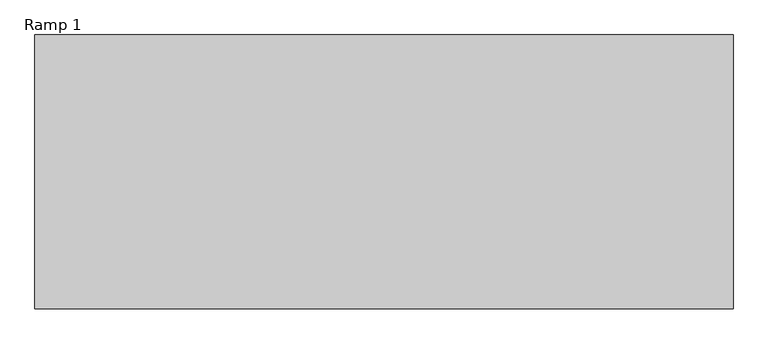
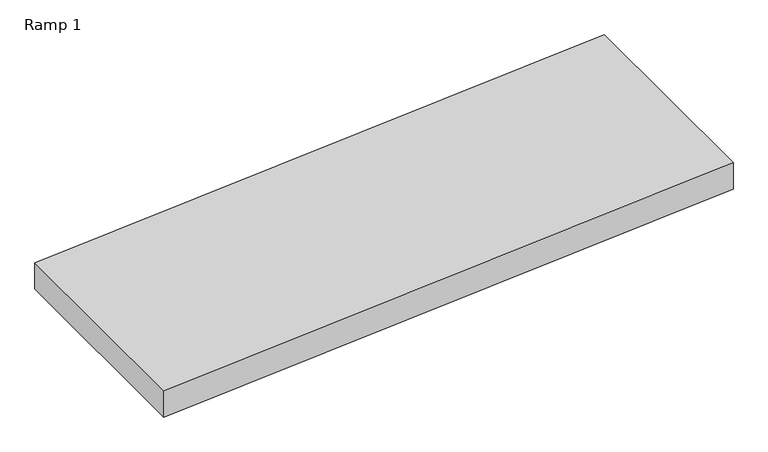
"""IFC4 building model written with IfcOpenShell, lengths in millimetres: ramp geometry, Ramp 1."""

import ifcopenshell
import ifcopenshell.guid

model = None  # the IFC model being written
_history = None  # IfcOwnerHistory: only IFC2X3 demands one
_inside = {}  # id of a spatial element -> (the spatial element, [elements in it])
_under = {}  # id of a project, library or spatial element -> (it, [spatial elements below it])
_declared = {}  # id of a project -> (the project, [libraries it declares])
_typed = {}  # id of a type object -> (the type object, [elements of that type])
_made_of = {}  # id of a material, layer set ... -> (it, [elements and type objects made of it])


def new_model(schema):
    """Start an empty IFC model of exactly this schema.

    Asked for "IFC4X3", IfcOpenShell would pick the latest addendum, in which some entities
    have other attributes; the version numbers below select the first issue.
    IFC2X3 requires an IfcOwnerHistory on every rooted entity: one is made here for all.
    """
    global model, _history
    if schema == "IFC4X3":
        model = ifcopenshell.file(schema_version=(4, 3, 0, 0))
    else:
        model = ifcopenshell.file(schema=schema)
    _inside.clear()
    _under.clear()
    _declared.clear()
    _typed.clear()
    _made_of.clear()
    _history = None
    if model.schema == "IFC2X3":
        org = make("IfcOrganization", Name="unknown")
        user = make(
            "IfcPersonAndOrganization",
            ThePerson=make("IfcPerson", FamilyName="unknown"),
            TheOrganization=org,
        )
        app = make(
            "IfcApplication",
            ApplicationDeveloper=org,
            Version="unknown",
            ApplicationFullName="unknown",
            ApplicationIdentifier="unknown",
        )
        _history = make(
            "IfcOwnerHistory",
            OwningUser=user,
            OwningApplication=app,
            ChangeAction="ADDED",
            CreationDate=0,
        )
    return model


def make(cls, **values):
    """One entity of the class cls with the attributes given. An attribute that is None is left unset."""
    return model.create_entity(
        cls, **{name: value for name, value in values.items() if value is not None}
    )


def rooted(cls, **values):
    """An entity with a GlobalId (a new one), such as an element, a storey or a relation."""
    return make(cls, GlobalId=ifcopenshell.guid.new(), OwnerHistory=_history, **values)


def si_unit(unit_type, name, prefix=None):
    """IfcSIUnit, for example si_unit("LENGTHUNIT", "METRE", prefix="MILLI")."""
    return make("IfcSIUnit", UnitType=unit_type, Prefix=prefix, Name=name)


def assignment(units):
    """IfcUnitAssignment: the units of a project."""
    return None if units is None else make("IfcUnitAssignment", Units=units)


def point(xyz):
    """IfcCartesianPoint."""
    return None if xyz is None else make("IfcCartesianPoint", Coordinates=xyz)


def direction(xyz):
    """IfcDirection."""
    return None if xyz is None else make("IfcDirection", DirectionRatios=xyz)


def frame(location, z_axis=None, x_axis=None):
    """IfcAxis2Placement3D, a coordinate frame: its origin and axes. An axis left out is left unset."""
    return make(
        "IfcAxis2Placement3D",
        Location=point(location),
        Axis=direction(z_axis),
        RefDirection=direction(x_axis),
    )


def origin():
    """The frame at (0, 0, 0) with its axes left unset."""
    return frame((0.0, 0.0, 0.0))


def place(relative_to, where):
    """IfcLocalPlacement: puts the frame where relative to a parent placement (None: the world)."""
    return make(
        "IfcLocalPlacement", PlacementRelTo=relative_to, RelativePlacement=where
    )


def context(
    kind, dimensions, precision=None, world=None, true_north=None, identifier=None
):
    """IfcGeometricRepresentationContext, for example the 3D "Model" context."""
    return make(
        "IfcGeometricRepresentationContext",
        ContextIdentifier=identifier,
        ContextType=kind,
        CoordinateSpaceDimension=dimensions,
        Precision=precision,
        WorldCoordinateSystem=world,
        TrueNorth=true_north,
    )


def project(units=None, contexts=None):
    """IfcProject with its units and contexts."""
    return rooted(
        "IfcProject",
        Name="project",
        RepresentationContexts=contexts,
        UnitsInContext=assignment(units),
    )


def spatial(cls, under=None, at=None, **own):
    """A site, building, storey or space (cls), placed at a placement, below another one or the project."""
    s = rooted(cls, ObjectPlacement=at, **own)
    if under is not None:
        _under.setdefault(under.id(), (under, []))[1].append(s)
    return s


def polyline(points):
    """IfcPolyline through the points."""
    return make("IfcPolyline", Points=[point(p) for p in points])


def outline(outer, holes=None, kind="AREA"):
    """IfcArbitraryClosedProfileDef: a profile drawn as a closed curve; with holes, ...WithVoids."""
    if holes is None:
        return make("IfcArbitraryClosedProfileDef", ProfileType=kind, OuterCurve=outer)
    return make(
        "IfcArbitraryProfileDefWithVoids",
        ProfileType=kind,
        OuterCurve=outer,
        InnerCurves=holes,
    )


def extrude(swept, where, along, depth):
    """IfcExtrudedAreaSolid: the profile swept, set in the frame where, extruded along a direction by depth."""
    return make(
        "IfcExtrudedAreaSolid",
        SweptArea=swept,
        Position=where,
        ExtrudedDirection=direction(along),
        Depth=depth,
    )


def shape(context_of_items, identifier, shape_type, items):
    """IfcShapeRepresentation: the items that make up one representation, for example the "Body"."""
    return make(
        "IfcShapeRepresentation",
        ContextOfItems=context_of_items,
        RepresentationIdentifier=identifier,
        RepresentationType=shape_type,
        Items=items,
    )


def source(mapping_origin, context_of_items, identifier, shape_type, items):
    """IfcRepresentationMap: a shape defined once, which mapped items show again and again."""
    return make(
        "IfcRepresentationMap",
        MappingOrigin=mapping_origin,
        MappedRepresentation=shape(context_of_items, identifier, shape_type, items),
    )


def transform(
    local_origin,
    x_axis=None,
    y_axis=None,
    z_axis=None,
    scale=None,
    scale2=None,
    scale3=None,
    uniform=True,
):
    """IfcCartesianTransformationOperator3D, or its non-uniform kind. x_axis, y_axis, z_axis: its Axis1, 2, 3."""
    if uniform:
        return make(
            "IfcCartesianTransformationOperator3D",
            Axis1=direction(x_axis),
            Axis2=direction(y_axis),
            LocalOrigin=point(local_origin),
            Scale=scale,
            Axis3=direction(z_axis),
        )
    return make(
        "IfcCartesianTransformationOperator3DnonUniform",
        Axis1=direction(x_axis),
        Axis2=direction(y_axis),
        LocalOrigin=point(local_origin),
        Scale=scale,
        Axis3=direction(z_axis),
        Scale2=scale2,
        Scale3=scale3,
    )


def mapped(mapping_source, mapping_target):
    """IfcMappedItem: shows the shape of a source again, moved by a transform."""
    return make(
        "IfcMappedItem", MappingSource=mapping_source, MappingTarget=mapping_target
    )


def made_of(thing, what):
    """Note that an element or type object is made of a material, layer set ...; save() writes the relation."""
    if what is not None:
        _made_of.setdefault(what.id(), (what, []))[1].append(thing)
    return thing


def element(
    cls,
    number,
    at=None,
    inside=None,
    cuts=None,
    type_object=None,
    material=None,
    context=None,
    identifier="Body",
    shape_type=None,
    held_by="IfcProductDefinitionShape",
    body=None,
    shapes=None,
    **own,
):
    """One element of the class cls, such as IfcWall. Its Tag is "e" and its number.

    at: its placement. inside: the storey or other place that contains it. cuts: it is an
    opening in that element (IfcRelVoidsElement). A single representation is given by context,
    identifier, shape_type and body (its items); several are given by shapes. held_by: the class
    of the entity that holds the representations. save() writes the other relations.
    """
    e = rooted(cls, Tag="e%d" % number, ObjectPlacement=at, **own)
    if body is not None:
        shapes = [shape(context, identifier, shape_type, body)]
    if shapes is not None:
        e.Representation = make(held_by, Representations=shapes)
    if inside is not None:
        _inside.setdefault(inside.id(), (inside, []))[1].append(e)
    if cuts is not None:
        rooted(
            "IfcRelVoidsElement", RelatingBuildingElement=cuts, RelatedOpeningElement=e
        )
    if type_object is not None:
        _typed.setdefault(type_object.id(), (type_object, []))[1].append(e)
    return made_of(e, material)


def aggregate(whole, parts):
    """IfcRelAggregates: a whole, such as a stair, and the parts it consists of."""
    return rooted("IfcRelAggregates", RelatingObject=whole, RelatedObjects=parts)


def save(model, path):
    """Write the relations noted so far, then the file.

    IfcRelAggregates (storeys below a building ...), IfcRelContainedInSpatialStructure (elements
    in a storey), IfcRelDefinesByType, IfcRelAssociatesMaterial and IfcRelDeclares: one each for
    every whole, place, type object, material and project.
    """
    for whole, parts in _under.values():
        aggregate(whole, parts)
    for where, things in _inside.values():
        rooted(
            "IfcRelContainedInSpatialStructure",
            RelatedElements=things,
            RelatingStructure=where,
        )
    for kind, things in _typed.values():
        rooted("IfcRelDefinesByType", RelatedObjects=things, RelatingType=kind)
    for what, things in _made_of.values():
        rooted("IfcRelAssociatesMaterial", RelatedObjects=things, RelatingMaterial=what)
    for by, libraries in _declared.values():
        rooted("IfcRelDeclares", RelatingContext=by, RelatedDefinitions=libraries)
    model.write(path)


def ramp_1_ce501800(model_context):
    return source(origin(), model_context, "Body", "SweptSolid", [
        extrude(outline(polyline([(0.0, -7500.2064028), (-225.0, -10560.2064028), (-375.4049465, -10560.2064028), (-150.4049465, -7500.2064028), (0.0, -7500.2064028)])), frame((0.0, -1636.162817, 0.0), z_axis=(0.0, 1.0, 0.0), x_axis=(0.0, 0.0, 1.0)), (0.0, 0.0, 1.0), 1200.0),
    ])


if __name__ == "__main__":
    model = new_model("IFC4")
    model_context = context("Model", 3, world=origin())
    ifc_project = project(units=[si_unit("LENGTHUNIT", "METRE", prefix="MILLI")], contexts=[model_context])
    site = spatial("IfcSite", under=ifc_project)
    building = spatial("IfcBuilding", under=site)
    placement = place(None, origin())
    ramp_1_shape = ramp_1_ce501800(model_context)
    element("IfcRamp", 1, ObjectType="Ramp 1", at=placement, inside=building, context=model_context, shape_type="MappedRepresentation", body=[
        mapped(ramp_1_shape, transform((0.0, 0.0, 0.0), x_axis=(1.0, 0.0, 0.0), y_axis=(0.0, 1.0, 0.0), z_axis=(0.0, 0.0, 1.0))),
    ])
    save(model, "model.ifc")

# Revit data of these elements
# Element 1 (IfcRamp, "Ramp 1")
#   Materials on its faces: "Concrete, Cast In Situ"
# Materials
#   "Concrete, Cast In Situ": class "Concrete", colour RGB 192 192 192, transparency 0, Keynote = "F30/110", Description = "physical material", Cost = 0
